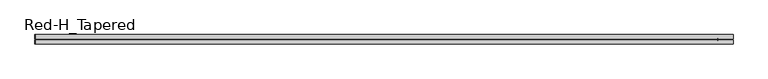
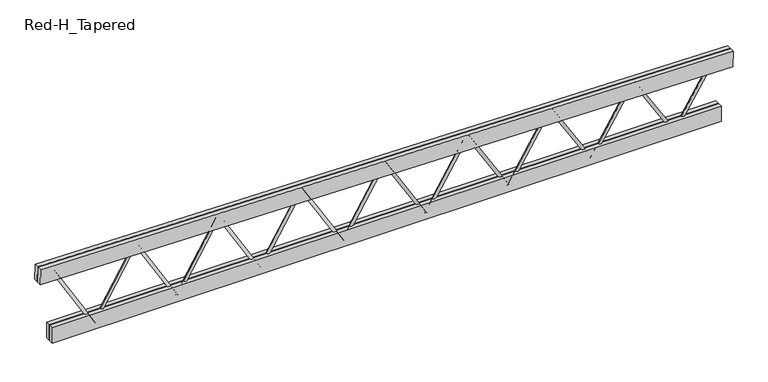
"""IFC4 building model written with IfcOpenShell, lengths in millimetres: beam geometry, Construction_Frames_RedBuilt_Openweb_Red-H_Tapered : Red-H_Tapered."""

import ifcopenshell
import ifcopenshell.guid

model = None  # the IFC model being written
_history = None  # IfcOwnerHistory: only IFC2X3 demands one
_inside = {}  # id of a spatial element -> (the spatial element, [elements in it])
_under = {}  # id of a project, library or spatial element -> (it, [spatial elements below it])
_declared = {}  # id of a project -> (the project, [libraries it declares])
_typed = {}  # id of a type object -> (the type object, [elements of that type])
_made_of = {}  # id of a material, layer set ... -> (it, [elements and type objects made of it])


def new_model(schema):
    """Start an empty IFC model of exactly this schema.

    Asked for "IFC4X3", IfcOpenShell would pick the latest addendum, in which some entities
    have other attributes; the version numbers below select the first issue.
    IFC2X3 requires an IfcOwnerHistory on every rooted entity: one is made here for all.
    """
    global model, _history
    if schema == "IFC4X3":
        model = ifcopenshell.file(schema_version=(4, 3, 0, 0))
    else:
        model = ifcopenshell.file(schema=schema)
    _inside.clear()
    _under.clear()
    _declared.clear()
    _typed.clear()
    _made_of.clear()
    _history = None
    if model.schema == "IFC2X3":
        org = make("IfcOrganization", Name="unknown")
        user = make(
            "IfcPersonAndOrganization",
            ThePerson=make("IfcPerson", FamilyName="unknown"),
            TheOrganization=org,
        )
        app = make(
            "IfcApplication",
            ApplicationDeveloper=org,
            Version="unknown",
            ApplicationFullName="unknown",
            ApplicationIdentifier="unknown",
        )
        _history = make(
            "IfcOwnerHistory",
            OwningUser=user,
            OwningApplication=app,
            ChangeAction="ADDED",
            CreationDate=0,
        )
    return model


def make(cls, **values):
    """One entity of the class cls with the attributes given. An attribute that is None is left unset."""
    return model.create_entity(
        cls, **{name: value for name, value in values.items() if value is not None}
    )


def rooted(cls, **values):
    """An entity with a GlobalId (a new one), such as an element, a storey or a relation."""
    return make(cls, GlobalId=ifcopenshell.guid.new(), OwnerHistory=_history, **values)


def si_unit(unit_type, name, prefix=None):
    """IfcSIUnit, for example si_unit("LENGTHUNIT", "METRE", prefix="MILLI")."""
    return make("IfcSIUnit", UnitType=unit_type, Prefix=prefix, Name=name)


def assignment(units):
    """IfcUnitAssignment: the units of a project."""
    return None if units is None else make("IfcUnitAssignment", Units=units)


def point(xyz):
    """IfcCartesianPoint."""
    return None if xyz is None else make("IfcCartesianPoint", Coordinates=xyz)


def direction(xyz):
    """IfcDirection."""
    return None if xyz is None else make("IfcDirection", DirectionRatios=xyz)


def frame(location, z_axis=None, x_axis=None):
    """IfcAxis2Placement3D, a coordinate frame: its origin and axes. An axis left out is left unset."""
    return make(
        "IfcAxis2Placement3D",
        Location=point(location),
        Axis=direction(z_axis),
        RefDirection=direction(x_axis),
    )


def frame_2d(location, x_axis=None):
    """IfcAxis2Placement2D, a coordinate frame in the plane: its origin and x axis."""
    return make(
        "IfcAxis2Placement2D", Location=point(location), RefDirection=direction(x_axis)
    )


def origin():
    """The frame at (0, 0, 0) with its axes left unset."""
    return frame((0.0, 0.0, 0.0))


def origin_2d():
    """The frame at (0, 0) in the plane with its x axis left unset."""
    return frame_2d((0.0, 0.0))


def place(relative_to, where):
    """IfcLocalPlacement: puts the frame where relative to a parent placement (None: the world)."""
    return make(
        "IfcLocalPlacement", PlacementRelTo=relative_to, RelativePlacement=where
    )


def context(
    kind, dimensions, precision=None, world=None, true_north=None, identifier=None
):
    """IfcGeometricRepresentationContext, for example the 3D "Model" context."""
    return make(
        "IfcGeometricRepresentationContext",
        ContextIdentifier=identifier,
        ContextType=kind,
        CoordinateSpaceDimension=dimensions,
        Precision=precision,
        WorldCoordinateSystem=world,
        TrueNorth=true_north,
    )


def project(units=None, contexts=None):
    """IfcProject with its units and contexts."""
    return rooted(
        "IfcProject",
        Name="project",
        RepresentationContexts=contexts,
        UnitsInContext=assignment(units),
    )


def spatial(cls, under=None, at=None, **own):
    """A site, building, storey or space (cls), placed at a placement, below another one or the project."""
    s = rooted(cls, ObjectPlacement=at, **own)
    if under is not None:
        _under.setdefault(under.id(), (under, []))[1].append(s)
    return s


def polyline(points):
    """IfcPolyline through the points."""
    return make("IfcPolyline", Points=[point(p) for p in points])


def circle_curve(where, radius):
    """IfcCircle in the frame where."""
    return make("IfcCircle", Position=where, Radius=radius)


def trimmed(basis, trim1, trim2, sense, master):
    """IfcTrimmedCurve: the piece of a basis curve between two trims."""
    return make(
        "IfcTrimmedCurve",
        BasisCurve=basis,
        Trim1=trim1,
        Trim2=trim2,
        SenseAgreement=sense,
        MasterRepresentation=master,
    )


def segment(curve, same_sense, transition):
    """IfcCompositeCurveSegment."""
    return make(
        "IfcCompositeCurveSegment",
        Transition=transition,
        SameSense=same_sense,
        ParentCurve=curve,
    )


def composite_curve(segments, self_intersect=None):
    """IfcCompositeCurve: segments joined end to end."""
    return make("IfcCompositeCurve", Segments=segments, SelfIntersect=self_intersect)


def outline(outer, holes=None, kind="AREA"):
    """IfcArbitraryClosedProfileDef: a profile drawn as a closed curve; with holes, ...WithVoids."""
    if holes is None:
        return make("IfcArbitraryClosedProfileDef", ProfileType=kind, OuterCurve=outer)
    return make(
        "IfcArbitraryProfileDefWithVoids",
        ProfileType=kind,
        OuterCurve=outer,
        InnerCurves=holes,
    )


def extrude(swept, where, along, depth):
    """IfcExtrudedAreaSolid: the profile swept, set in the frame where, extruded along a direction by depth."""
    return make(
        "IfcExtrudedAreaSolid",
        SweptArea=swept,
        Position=where,
        ExtrudedDirection=direction(along),
        Depth=depth,
    )


def shape(context_of_items, identifier, shape_type, items):
    """IfcShapeRepresentation: the items that make up one representation, for example the "Body"."""
    return make(
        "IfcShapeRepresentation",
        ContextOfItems=context_of_items,
        RepresentationIdentifier=identifier,
        RepresentationType=shape_type,
        Items=items,
    )


def source(mapping_origin, context_of_items, identifier, shape_type, items):
    """IfcRepresentationMap: a shape defined once, which mapped items show again and again."""
    return make(
        "IfcRepresentationMap",
        MappingOrigin=mapping_origin,
        MappedRepresentation=shape(context_of_items, identifier, shape_type, items),
    )


def transform(
    local_origin,
    x_axis=None,
    y_axis=None,
    z_axis=None,
    scale=None,
    scale2=None,
    scale3=None,
    uniform=True,
):
    """IfcCartesianTransformationOperator3D, or its non-uniform kind. x_axis, y_axis, z_axis: its Axis1, 2, 3."""
    if uniform:
        return make(
            "IfcCartesianTransformationOperator3D",
            Axis1=direction(x_axis),
            Axis2=direction(y_axis),
            LocalOrigin=point(local_origin),
            Scale=scale,
            Axis3=direction(z_axis),
        )
    return make(
        "IfcCartesianTransformationOperator3DnonUniform",
        Axis1=direction(x_axis),
        Axis2=direction(y_axis),
        LocalOrigin=point(local_origin),
        Scale=scale,
        Axis3=direction(z_axis),
        Scale2=scale2,
        Scale3=scale3,
    )


def mapped(mapping_source, mapping_target):
    """IfcMappedItem: shows the shape of a source again, moved by a transform."""
    return make(
        "IfcMappedItem", MappingSource=mapping_source, MappingTarget=mapping_target
    )


def made_of(thing, what):
    """Note that an element or type object is made of a material, layer set ...; save() writes the relation."""
    if what is not None:
        _made_of.setdefault(what.id(), (what, []))[1].append(thing)
    return thing


def element(
    cls,
    number,
    at=None,
    inside=None,
    cuts=None,
    type_object=None,
    material=None,
    context=None,
    identifier="Body",
    shape_type=None,
    held_by="IfcProductDefinitionShape",
    body=None,
    shapes=None,
    **own,
):
    """One element of the class cls, such as IfcWall. Its Tag is "e" and its number.

    at: its placement. inside: the storey or other place that contains it. cuts: it is an
    opening in that element (IfcRelVoidsElement). A single representation is given by context,
    identifier, shape_type and body (its items); several are given by shapes. held_by: the class
    of the entity that holds the representations. save() writes the other relations.
    """
    e = rooted(cls, Tag="e%d" % number, ObjectPlacement=at, **own)
    if body is not None:
        shapes = [shape(context, identifier, shape_type, body)]
    if shapes is not None:
        e.Representation = make(held_by, Representations=shapes)
    if inside is not None:
        _inside.setdefault(inside.id(), (inside, []))[1].append(e)
    if cuts is not None:
        rooted(
            "IfcRelVoidsElement", RelatingBuildingElement=cuts, RelatedOpeningElement=e
        )
    if type_object is not None:
        _typed.setdefault(type_object.id(), (type_object, []))[1].append(e)
    return made_of(e, material)


def aggregate(whole, parts):
    """IfcRelAggregates: a whole, such as a stair, and the parts it consists of."""
    return rooted("IfcRelAggregates", RelatingObject=whole, RelatedObjects=parts)


def save(model, path):
    """Write the relations noted so far, then the file.

    IfcRelAggregates (storeys below a building ...), IfcRelContainedInSpatialStructure (elements
    in a storey), IfcRelDefinesByType, IfcRelAssociatesMaterial and IfcRelDeclares: one each for
    every whole, place, type object, material and project.
    """
    for whole, parts in _under.values():
        aggregate(whole, parts)
    for where, things in _inside.values():
        rooted(
            "IfcRelContainedInSpatialStructure",
            RelatedElements=things,
            RelatingStructure=where,
        )
    for kind, things in _typed.values():
        rooted("IfcRelDefinesByType", RelatedObjects=things, RelatingType=kind)
    for what, things in _made_of.values():
        rooted("IfcRelAssociatesMaterial", RelatedObjects=things, RelatingMaterial=what)
    for by, libraries in _declared.values():
        rooted("IfcRelDeclares", RelatingContext=by, RelatedDefinitions=libraries)
    model.write(path)


def red_h_tapered_6d79e80b(model_context):
    return source(origin(), model_context, "Body", "SweptSolid", [
        extrude(outline(composite_curve([segment(trimmed(circle_curve(origin_2d(), 12.7), [point((0.0, 12.7))], [point((0.0, -12.7))], False, "CARTESIAN"), True, "CONTINUOUS"), segment(trimmed(circle_curve(origin_2d(), 12.7), [point((0.0, -12.7))], [point((0.0, 12.7))], False, "CARTESIAN"), True, "CONTINUOUS")], self_intersect=False)), frame((2526.107324, 0.0, -367.0101562), z_axis=(0.5255382750472374, 0.0, 0.8507699580147235), x_axis=(0.0, -1.0, 0.0)), (0.0, 0.0, 1.0), 686.6721074),
        extrude(outline(composite_curve([segment(trimmed(circle_curve(origin_2d(), 12.7), [point((0.0, -12.7))], [point((0.0, 12.6999999))], False, "CARTESIAN"), True, "CONTINUOUS"), segment(trimmed(circle_curve(origin_2d(), 12.7), [point((0.0, 12.6999999))], [point((0.0, -12.7))], False, "CARTESIAN"), True, "CONTINUOUS")], self_intersect=False)), frame((2526.107324, 0.0, -367.0101562), z_axis=(-0.5229651633515324, 0.0, 0.8523540566693545), x_axis=(0.0, -1.0, 0.0)), (0.0, 0.0, 1.0), 690.0506958),
        extrude(outline(composite_curve([segment(trimmed(circle_curve(origin_2d(), 12.7), [point((0.0, 12.7))], [point((0.0, -12.6999999))], False, "CARTESIAN"), True, "CONTINUOUS"), segment(trimmed(circle_curve(origin_2d(), 12.7), [point((0.0, -12.6999999))], [point((0.0, 12.7))], False, "CARTESIAN"), True, "CONTINUOUS")], self_intersect=False)), frame((1804.3623743, 0.0, -367.0101562), z_axis=(0.5229651633515339, 0.0, 0.8523540566693536), x_axis=(0.0, -1.0, 0.0)), (0.0, 0.0, 1.0), 690.0506958),
        extrude(outline(composite_curve([segment(trimmed(circle_curve(origin_2d(), 12.7), [point((0.0, -12.7000001))], [point((0.0, 12.6999999))], False, "CARTESIAN"), True, "CONTINUOUS"), segment(trimmed(circle_curve(origin_2d(), 12.7), [point((0.0, 12.6999999))], [point((0.0, -12.7000001))], False, "CARTESIAN"), True, "CONTINUOUS")], self_intersect=False)), frame((1804.3623743, 0.0, -367.0101562), z_axis=(-0.5204124432875953, 0.0, 0.8539150360963529), x_axis=(0.0, -1.0, 0.0)), (0.0, 0.0, 1.0), 693.4355231),
        extrude(outline(composite_curve([segment(trimmed(circle_curve(origin_2d(), 12.7), [point((0.0, 12.7))], [point((0.0, -12.7))], False, "CARTESIAN"), True, "CONTINUOUS"), segment(trimmed(circle_curve(origin_2d(), 12.7), [point((0.0, -12.7))], [point((0.0, 12.7))], False, "CARTESIAN"), True, "CONTINUOUS")], self_intersect=False)), frame((1082.6174246, 0.0, -367.0101562), z_axis=(0.5204124432875943, 0.0, 0.8539150360963534), x_axis=(0.0, -1.0, 0.0)), (0.0, 0.0, 1.0), 693.4355231),
        extrude(outline(composite_curve([segment(trimmed(circle_curve(origin_2d(), 12.7), [point((0.0, -12.7000001))], [point((0.0, 12.7))], False, "CARTESIAN"), True, "CONTINUOUS"), segment(trimmed(circle_curve(origin_2d(), 12.7), [point((0.0, 12.7))], [point((0.0, -12.7000001))], False, "CARTESIAN"), True, "CONTINUOUS")], self_intersect=False)), frame((1082.6174246, 0.0, -367.0101562), z_axis=(-0.5178799538342008, 0.0, 0.855453302884901), x_axis=(0.0, -1.0, 0.0)), (0.0, 0.0, 1.0), 696.8264985),
        extrude(outline(composite_curve([segment(trimmed(circle_curve(origin_2d(), 12.7), [point((0.0, 12.7))], [point((0.0, -12.7))], False, "CARTESIAN"), True, "CONTINUOUS"), segment(trimmed(circle_curve(origin_2d(), 12.7), [point((0.0, -12.7))], [point((0.0, 12.7))], False, "CARTESIAN"), True, "CONTINUOUS")], self_intersect=False)), frame((360.8724749, 0.0, -367.0101562), z_axis=(0.5178799538342008, 0.0, 0.855453302884901), x_axis=(0.0, -1.0, 0.0)), (0.0, 0.0, 1.0), 696.8264985),
        extrude(outline(composite_curve([segment(trimmed(circle_curve(origin_2d(), 12.7), [point((0.0, -12.7000001))], [point((0.0, 12.6999999))], False, "CARTESIAN"), True, "CONTINUOUS"), segment(trimmed(circle_curve(origin_2d(), 12.7), [point((0.0, 12.6999999))], [point((0.0, -12.7000001))], False, "CARTESIAN"), True, "CONTINUOUS")], self_intersect=False)), frame((360.8724749, 0.0, -367.0101562), z_axis=(-0.5153675335242818, 0.0, 0.856969255801571), x_axis=(0.0, -1.0, 0.0)), (0.0, 0.0, 1.0), 700.2235325),
        extrude(outline(composite_curve([segment(trimmed(circle_curve(origin_2d(), 12.7), [point((0.0, -12.6999999))], [point((0.0, 12.7000001))], False, "CARTESIAN"), True, "CONTINUOUS"), segment(trimmed(circle_curve(origin_2d(), 12.7), [point((0.0, 12.7000001))], [point((0.0, -12.6999999))], False, "CARTESIAN"), True, "CONTINUOUS")], self_intersect=False)), frame((-360.8724749, 0.0, -367.0101562), z_axis=(0.5153675335242504, 0.0, 0.8569692558015899), x_axis=(0.0, -1.0, 0.0)), (0.0, 0.0, 1.0), 700.2235325),
        extrude(outline(composite_curve([segment(trimmed(circle_curve(origin_2d(), 12.7), [point((0.0, 12.7))], [point((0.0, -12.7))], False, "CARTESIAN"), True, "CONTINUOUS"), segment(trimmed(circle_curve(origin_2d(), 12.7), [point((0.0, -12.7))], [point((0.0, 12.7))], False, "CARTESIAN"), True, "CONTINUOUS")], self_intersect=False)), frame((-360.8724749, 0.0, -367.0101562), z_axis=(-0.5128750205463383, 0.0, 0.8584632859357428), x_axis=(0.0, -1.0, 0.0)), (0.0, 0.0, 1.0), 703.6265375),
        extrude(outline(composite_curve([segment(trimmed(circle_curve(origin_2d(), 12.7), [point((0.0, -12.6999999))], [point((0.0, 12.7000001))], False, "CARTESIAN"), True, "CONTINUOUS"), segment(trimmed(circle_curve(origin_2d(), 12.7), [point((0.0, 12.7000001))], [point((0.0, -12.6999999))], False, "CARTESIAN"), True, "CONTINUOUS")], self_intersect=False)), frame((-1082.6174246, 0.0, -367.0101562), z_axis=(0.5128750205463365, 0.0, 0.858463285935744), x_axis=(0.0, -1.0, 0.0)), (0.0, 0.0, 1.0), 703.6265375),
        extrude(outline(composite_curve([segment(trimmed(circle_curve(origin_2d(), 12.7), [point((0.0, 12.7))], [point((0.0, -12.7))], False, "CARTESIAN"), True, "CONTINUOUS"), segment(trimmed(circle_curve(origin_2d(), 12.7), [point((0.0, -12.7))], [point((0.0, 12.7))], False, "CARTESIAN"), True, "CONTINUOUS")], self_intersect=False)), frame((-1082.6174246, 0.0, -367.0101562), z_axis=(-0.5104022528410607, 0.0, 0.8599357768431141), x_axis=(0.0, -1.0, 0.0)), (0.0, 0.0, 1.0), 707.0354272),
        extrude(outline(composite_curve([segment(trimmed(circle_curve(origin_2d(), 12.7), [point((0.0, -12.7))], [point((0.0, 12.7000001))], False, "CARTESIAN"), True, "CONTINUOUS"), segment(trimmed(circle_curve(origin_2d(), 12.7), [point((0.0, 12.7000001))], [point((0.0, -12.7))], False, "CARTESIAN"), True, "CONTINUOUS")], self_intersect=False)), frame((-1804.3623743, 0.0, -367.0101562), z_axis=(0.510402252841074, 0.0, 0.8599357768431061), x_axis=(0.0, -1.0, 0.0)), (0.0, 0.0, 1.0), 707.0354272),
        extrude(outline(composite_curve([segment(trimmed(circle_curve(origin_2d(), 12.7), [point((0.0, 12.6999999))], [point((0.0, -12.7))], False, "CARTESIAN"), True, "CONTINUOUS"), segment(trimmed(circle_curve(origin_2d(), 12.7), [point((0.0, -12.7))], [point((0.0, 12.6999999))], False, "CARTESIAN"), True, "CONTINUOUS")], self_intersect=False)), frame((-1804.3623743, 0.0, -367.0101562), z_axis=(-0.5079490681928376, 0.0, 0.8613871046875662), x_axis=(0.0, -1.0, 0.0)), (0.0, 0.0, 1.0), 710.4501169),
        extrude(outline(composite_curve([segment(trimmed(circle_curve(origin_2d(), 12.7), [point((0.0, -12.6999999))], [point((0.0, 12.7))], False, "CARTESIAN"), True, "CONTINUOUS"), segment(trimmed(circle_curve(origin_2d(), 12.7), [point((0.0, 12.7))], [point((0.0, -12.6999999))], False, "CARTESIAN"), True, "CONTINUOUS")], self_intersect=False)), frame((-2526.107324, 0.0, -367.0101562), z_axis=(0.5079490681928277, 0.0, 0.861387104687572), x_axis=(0.0, -1.0, 0.0)), (0.0, 0.0, 1.0), 710.4501169),
        extrude(outline(composite_curve([segment(trimmed(circle_curve(origin_2d(), 12.7), [point((0.0, 12.7))], [point((0.0, -12.7))], False, "CARTESIAN"), True, "CONTINUOUS"), segment(trimmed(circle_curve(origin_2d(), 12.7), [point((0.0, -12.7))], [point((0.0, 12.7))], False, "CARTESIAN"), True, "CONTINUOUS")], self_intersect=False)), frame((-2526.107324, 0.0, -367.0101562), z_axis=(-0.5055153043168177, 0.0, 0.8628176383810633), x_axis=(0.0, -1.0, 0.0)), (0.0, 0.0, 1.0), 713.8705234),
        extrude(outline(polyline([(-2912.3797989, -41.275), (-2912.3797989, -3.175), (2912.3797989, -3.175), (2912.3797989, -41.275), (-2912.3797989, -41.275)])), frame((0.0, 0.0, -386.0601562), z_axis=(0.0, 0.0, 1.0), x_axis=(1.0, 0.0, 0.0)), (0.0, 0.0, 1.0), 139.7),
        extrude(outline(polyline([(-2912.3797989, 3.175), (-2912.3797989, 41.275), (2912.3797989, 41.275), (2912.3797989, 3.175), (-2912.3797989, 3.175)])), frame((0.0, 0.0, -386.0601562), z_axis=(0.0, 0.0, 1.0), x_axis=(1.0, 0.0, 0.0)), (0.0, 0.0, 1.0), 139.7),
        extrude(outline(polyline([(0.0, -38.1), (0.0, 0.0), (6028.8157603, 0.0), (6028.8157603, -38.1), (0.0, -38.1)])), frame((-3016.3340788, -3.175, 185.4596828), z_axis=(0.016852397558582144, 0.0, 0.9998579882645973), x_axis=(0.9998579882645973, 0.0, -0.016852397558582144)), (0.0, 0.0, 1.0), 139.7),
        extrude(outline(polyline([(0.0, -38.1), (0.0, 0.0), (6028.8157603, 0.0), (6028.8157603, -38.1), (0.0, -38.1)])), frame((-3016.3340788, 41.275, 185.4596828), z_axis=(0.016852397558582144, 0.0, 0.9998579882645973), x_axis=(0.9998579882645973, 0.0, -0.016852397558582144)), (0.0, 0.0, 1.0), 139.7),
    ])


if __name__ == "__main__":
    model = new_model("IFC4")
    model_context = context("Model", 3, world=origin())
    ifc_project = project(units=[si_unit("LENGTHUNIT", "METRE", prefix="MILLI")], contexts=[model_context])
    site = spatial("IfcSite", under=ifc_project)
    building = spatial("IfcBuilding", under=site)
    placement = place(None, origin())
    red_h_tapered_shape = red_h_tapered_6d79e80b(model_context)
    element("IfcBeam", 1, ObjectType="Construction_Frames_RedBuilt_Openweb_Red-H_Tapered : Red-H_Tapered", at=placement, inside=building, context=model_context, shape_type="MappedRepresentation", body=[
        mapped(red_h_tapered_shape, transform((0.0, 0.0, 0.0), x_axis=(1.0, 0.0, 0.0), y_axis=(0.0, 1.0, 0.0), z_axis=(0.0, 0.0, 1.0))),
    ])
    save(model, "model.ifc")

# Revit data of these elements
# Type "Construction_Frames_RedBuilt_Openweb_Red-H_Tapered : Red-H_Tapered"
#   Youtube clip = ""
#   Weight Net (Kg) = "0"
#   Webs = "Up to 2\" diameter tubular steel"
#   Uniformat II Description = ""
#   Uniformat II Code = ""
#   Uniclass 2015 Name = "Softwood trusses"
#   Uniclass 2015 Code = "Pr_20_85_90_81"
#   Uniclass 2.0 Description = "Structural Framing Systems"
#   Uniclass 2.0 Code = "SS-15-10-75"
#   Uniclass 1.4 Description = "Trusses"
#   Uniclass 1.4 Code = "L3523"
#   UNSPSC Code = "30103606"
#   Technical description = "http://www.redbuilt.com/reference/literature-and-other-resources"
#   Region South America = "None"
#   Region Oceania = "None"
#   Region North America = "US"
#   Region Middle East = "None"
#   Region Europe = "None"
#   Region Asia = "None"
#   Region Antarctica = "None"
#   Region Africa = "None"
#   QR code = "http://bimobject.com/redbuilt/product/redbuilt-0003"
#   Product url = "http://www.redbuilt.com/products/default.aspx?id=2"
#   Product group = "Wood Trusses"
#   Product family = "Construction"
#   Product data url = "https://bimobject.com/redbuilt/product/redbuilt-0003"
#   Product certification = ""
#   Product SKU = "redbuilt-0003"
#   Product Page URL = "http://www.redbuilt.com/commercial-systems/red-m-red-h-open-web-trusses"
#   Product Guid = "2c5793f2-6ffb-4665-b825-cf90c048e711"
#   Product Documentation Link = "http://www.redbuilt.com/documents/OW_Guide_2017_07_LowRes_wLinks.pdf"
#   OmniClass Description = "Wood Trusses"
#   OmniClass Code = "23-13 35 19 13 17"
#   NBS Reference Description = ""
#   NBS Reference Code = ""
#   Material secondary = "Steel"
#   Material main = "CHARRED WOOD"
#   Masterformat 2014 Description = "Metal-Web Wood Joists"
#   Masterformat 2014 Code = "06 17 36"
#   Manufacturer name = "RedBuilt"
#   Manufacturer country = "United States"
#   Installation instructions = "http://www.redbuilt.com/documents/Installation_Sheets_Open-Web.pdf"
#   IFC Classification = ""
#   EAN code = ""
#   Design country = "United States"
#   Product Information = "http://redbuilt.com/products/default.aspx?id=2"
#   Model = "Red-H-Tapered"
#   Manufacturer URL = "http://redbuilt.com/"
#   Manufacturer = "RedBuilt™"
#   Description = "Open Web Truss"
#   Date of publishing = "8/17/2010"
#   Contact us = "http://redbuilt.com/contact/"
#   Chords = "Double 1½\" x 5½\" MSR lumber"
#   COBIe Type Category = ""
#   Brand url = "http://www.redbuilt.com"
#   BIMobject main category code = "construction"
#   BIMobject main category = "Construction"
#   BIMobject category code = "construction-frames-trusses"
#   BIMobject category = "Frames & Trusses"
#   Web Radius = 0' - 0 1/2"
#   Web Layout Offset Start [instance default] = 0' - 5"
#   Web Layout Offset End [instance default] = 0' - 5"
#   Web Diameter = 0' - 1"
#   TotalLength [instance default] = 20' - 0"
#   Span Minimum = 4' - 0"
#   Span Maximum = 70' - 0"
#   Span Limit [instance default] = 20' - 0"
#   Nominal width = 0' - 0"
#   Nominal height = 0' - 0"
#   Inner Depth Top [instance default] = 0' - 2.76372"
#   Depth Start [instance default] = 6' - 0"
#   Top Chord Length [instance default] = 20' - 1.19701"
#   TC Extension Start Aux [instance default] = 0' - 0"
#   TC Extension End Aux [instance default] = 0' - 0"
#   T-B Chord Length Difference L [instance default] = 0' - 4"
#   T-B Chord Length Difference [instance default] = 0' - 4"
#   Height 2 [instance default] = 6' - 0"
#   Depth Minimum at Wall = 2' - 0"
#   Depth Maximum at Wall = 6' - 0"
#   Depth Lower End [instance default] = 2' - 0"
#   Depth Higher End [instance default] = 6' - 0"
#   Depth End [instance default] = 2' - 0"
#   Depth 2 [instance default] = 2' - 0"
#   Chord Width = 0' - 3 1/4"
#   Chord Thickness = 0' - 1 1/2"
#   Chord Depth = 0' - 5 1/2"
#   Offset Start [instance default] = 0' - 0"
#   TC Extension Start [instance default] = 0' - 0"
#   End Panel = 0' - 5"
#   Offset End [instance default] = 0' - 0"
#   TC Extension End [instance default] = 0' - 0"
#   Length [instance default] = 20' - 0"
#   Angle [instance default] = 5.71059°
#   Span Limit Warning [instance default] = no
#   Edition number = 1
#   Top Bearing Start [instance default] = yes
#   Top Bearing End [instance default] = yes
#   Bottom Bearing Start [instance default] = no
#   Bottom Bearing End [instance default] = no
#   8 Panels [instance default] = yes
#   16 Panels [instance default] = no
#   12 Panels [instance default] = no
#   Web Material = RedBuilt-Steel, Galvanized
#   Clip Material = RedBuilt-Steel, Galvanized
#   Chords Material = WOOD-OAKFIRE
#   URL = ""
#   Assembly Code = ""
# Element 1 (IfcBeam, "Construction_Frames_RedBuilt_Openweb_Red-H_Tapered : Red-H_Tapered")
#   TotalLength = 19' - 9.32124"
#   Span Limit = 19' - 9.32124"
#   Inner Depth Top = 0' - 2.75039"
#   Depth Start = 5' - 0"
#   Top Chord Length = 19' - 9.35495"
#   Height 2 = 5' - 0"
#   Depth Higher End = 5' - 0"
#   Depth 2 = 0' - 4"
#   Angle = 0.965617°
#   Materials on its faces: "RedBuilt-Steel, Galvanized", "WOOD-OAKFIRE"
# Materials
#   "RedBuilt-Steel, Galvanized": class "Metal", colour RGB 164 172 176, transparency 0, Manufacturer = "RedBuilt. LLC", Comments = "Openweb Metal Web", URL = "http://www.redbuilt.com/", Description = "Galvanized steel", Cost = 0
#   "WOOD-OAKFIRE": class "Wood", colour RGB 198 202 183, transparency 0, Description = "Generic wood", Cost = 0
